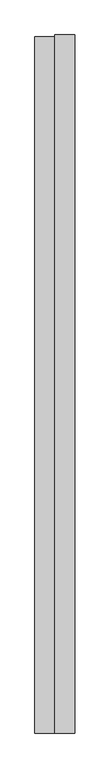
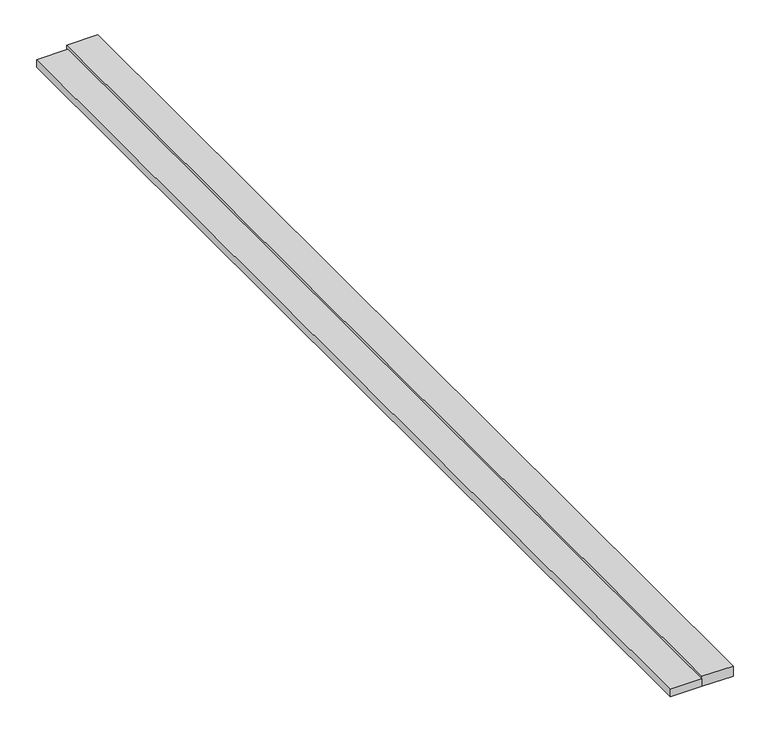
"""IFC4 building model written with IfcOpenShell, lengths in millimetres: proxy geometry, Generic Models 3:Generic Models 1:6:Generic Models 1:6 : Generic Models 3:Generic Models 1:300625:350611:Generic Models 1:6:Generic Models 1:6 : Generic Models 3:Generic Models 1:300625:350611 : Generic Models 3:Generic Models 1:6:Generic Models 1:6 : Generic Models 3:Generic Models 1:300625:350611:9 : Generic Models 3:Generic Models 1:6:Generic Models 1:6 : Generic Models 3:Generic Models 1:300625:350611:Generic Models 1:6:Generic Models 1:6 : Generic Models 3:Generic Models 1:300625:350611 : Generic Models 3:Generic Models 1:6:Generic Models 1:6 : Generic Models 3:Generic Models 1:300625:350611:301824."""

from ifc_helpers import new_model, si_unit, frame, origin, place, context, project, spatial, polyline, outline, extrude, source, transform, mapped, element, save


def generic_models_75cca51a(model_context):
    return source(origin(), model_context, "Body", "SweptSolid", [
        extrude(outline(polyline([(560225.9617239, -543189.8663841), (560295.7010166, -543189.8663841), (560295.7010166, -545628.2663841), (560225.9617239, -545628.2663841), (560225.9617239, -543189.8663841)])), frame((0.0, 0.0, 1.3647904), z_axis=(0.0, 0.0, 1.0), x_axis=(1.0, 0.0, 0.0)), (0.0, 0.0, 1.0), 17.6585659),
        extrude(outline(polyline([(560296.2248072, -543183.5163841), (560365.6617239, -543183.5163841), (560365.6617239, -545628.2663841), (560296.2248072, -545628.2663841), (560296.2248072, -543183.5163841)])), frame((0.0, 0.0, 1.3647904), z_axis=(0.0, 0.0, 1.0), x_axis=(1.0, 0.0, 0.0)), (0.0, 0.0, 1.0), 23.478574),
    ])


if __name__ == "__main__":
    model = new_model("IFC4")
    model_context = context("Model", 3, world=origin())
    ifc_project = project(units=[si_unit("LENGTHUNIT", "METRE", prefix="MILLI")], contexts=[model_context])
    site = spatial("IfcSite", under=ifc_project)
    building = spatial("IfcBuilding", under=site)
    placement = place(None, origin())
    generic_models_shape = generic_models_75cca51a(model_context)
    element("IfcBuildingElementProxy", 1, Name="Generic Models 3:Generic Models 1:6:Generic Models 1:6 : Generic Models 3:Generic Models 1:300625:350611:Generic Models 1:6:Generic Models 1:6 : Generic Models 3:Generic Models 1:300625:350611 : Generic Models 3:Generic Models 1:6:Generic Models 1:6 : Generic Models 3:Generic Models 1:300625:350611:9 : Generic Models 3:Generic Models 1:6:Generic Models 1:6 : Generic Models 3:Generic Models 1:300625:350611:Generic Models 1:6:Generic Models 1:6 : Generic Models 3:Generic Models 1:300625:350611 : Generic Models 3:Generic Models 1:6:Generic Models 1:6 : Generic Models 3:Generic Models 1:300625:350611:301824", ObjectType="Generic Models 3:Generic Models 1:6:Generic Models 1:6 : Generic Models 3:Generic Models 1:300625:350611:Generic Models 1:6:Generic Models 1:6 : Generic Models 3:Generic Models 1:300625:350611 : Generic Models 3:Generic Models 1:6:Generic Models 1:6 : Generic Models 3:Generic Models 1:300625:350611:9 : Generic Models 3:Generic Models 1:6:Generic Models 1:6 : Generic Models 3:Generic Models 1:300625:350611:Generic Models 1:6:Generic Models 1:6 : Generic Models 3:Generic Models 1:300625:350611 : Generic Models 3:Generic Models 1:6:Generic Models 1:6 : Generic Models 3:Generic Models 1:300625:350611:301824", at=placement, inside=building, context=model_context, shape_type="MappedRepresentation", body=[
        mapped(generic_models_shape, transform((0.0, 0.0, 0.0), x_axis=(1.0, 0.0, 0.0), y_axis=(0.0, 1.0, 0.0), z_axis=(0.0, 0.0, 1.0))),
    ])
    save(model, "model.ifc")

# Revit data of these elements
# Type "Generic Models 3:Generic Models 1:6:Generic Models 1:6 : Generic Models 3:Generic Models 1:300625:350611:Generic Models 1:6:Generic Models 1:6 : Generic Models 3:Generic Models 1:300625:350611 : Generic Models 3:Generic Models 1:6:Generic Models 1:6 : Generic Models 3:Generic Models 1:300625:350611:9 : Generic Models 3:Generic Models 1:6:Generic Models 1:6 : Generic Models 3:Generic Models 1:300625:350611:Generic Models 1:6:Generic Models 1:6 : Generic Models 3:Generic Models 1:300625:350611 : Generic Models 3:Generic Models 1:6:Generic Models 1:6 : Generic Models 3:Generic Models 1:300625:350611:301824"
#   NameOverride = "Generic Models 3:Generic Models 1:6:Generic Models 1:6 : Generic Models 3:Generic Models 1:300625:350611:Generic Models 1:6:Generic Models 1:6 : Generic Models 3:Generic Models 1:300625:350611 : Generic Models 3:Generic Models 1:6:Generic Models 1:6 : Generic Models 3:Generic Models 1:300625:350611:301824"
#   ObjectTypeOverride = "Generic Models 1:6:Generic Models 1:6 : Generic Models 3:Generic Models 1:300625:350611 : Generic Models 3:Generic Models 1:6:Generic Models 1:6 : Generic Models 3:Generic Models 1:300625:350611"
#   Reference = "Generic Models 1"
#   Tag = "301824"
# Element 1 (IfcBuildingElementProxy, "Generic Models 3:Generic Models 1:6:Generic Models 1:6 : Generic Models 3:Generic Models 1:300625:350611:Generic Models 1:6:Generic Models 1:6 : Generic Models 3:Generic Models 1:300625:350611 : Generic Models 3:Generic Models 1:6:Generic Models 1:6 : Generic Models 3:Generic Models 1:300625:350611:9 : Generic Models 3:Generic Models 1:6:Generic Models 1:6 : Generic Models 3:Generic Models 1:300625:350611:Generic Models 1:6:Generic Models 1:6 : Generic Models 3:Generic Models 1:300625:350611 : Generic Models 3:Generic Models 1:6:Generic Models 1:6 : Generic Models 3:Generic Models 1:300625:350611:301824")
#   Materials on its faces: "EXTRUDED POLYSTYRENE (XPS) RIGID FOAM INSULATION (FOAMULAR® 250 OR SIMILAR)"
# Materials
#   "EXTRUDED POLYSTYRENE (XPS) RIGID FOAM INSULATION (FOAMULAR® 250 OR SIMILAR)": class "Unassigned", colour RGB 247 185 194, transparency 0, Cost = 0
